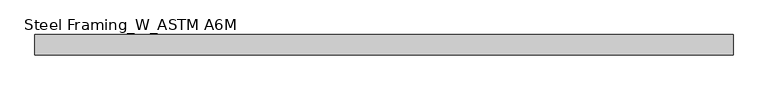
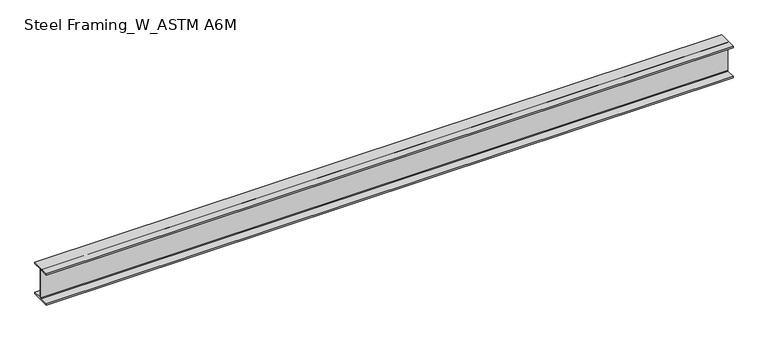
"""IFC4 building model written with IfcOpenShell, lengths in millimetres: beam geometry, Steel Framing_W_ASTM A6M : H_SB_AR_S02_W460x128_B1."""

from ifc_helpers import new_model, si_unit, point, frame, frame_2d, origin, place, context, project, spatial, polyline, circle_curve, trimmed, segment, composite_curve, outline, extrude, source, transform, mapped, element, save


def steel_framing_w_astm_a6m_6918b6cf(model_context):
    return source(origin(), model_context, "Body", "SweptSolid", [
        extrude(outline(composite_curve([segment(polyline([(141.0, -213.9), (141.0, -233.5), (-141.0, -233.5), (-141.0, -213.9), (-16.2, -213.9)]), True, "CONTINUOUS"), segment(trimmed(circle_curve(frame_2d((-16.2, -203.8)), 10.1), [point((-16.2, -213.9))], [point((-6.1, -203.8))], True, "CARTESIAN"), True, "CONTINUOUS"), segment(polyline([(-6.1, -203.8), (-6.1, 203.8)]), True, "CONTINUOUS"), segment(trimmed(circle_curve(frame_2d((-16.2, 203.8)), 10.1), [point((-6.1, 203.8))], [point((-16.2, 213.9))], True, "CARTESIAN"), True, "CONTINUOUS"), segment(polyline([(-16.2, 213.9), (-141.0, 213.9), (-141.0, 233.5), (141.0, 233.5), (141.0, 213.9), (16.2, 213.9)]), True, "CONTINUOUS"), segment(trimmed(circle_curve(frame_2d((16.2, 203.8)), 10.1), [point((16.2, 213.9))], [point((6.1, 203.8))], True, "CARTESIAN"), True, "CONTINUOUS"), segment(polyline([(6.1, 203.8), (6.1, -203.8)]), True, "CONTINUOUS"), segment(trimmed(circle_curve(frame_2d((16.2, -203.8)), 10.1), [point((6.1, -203.8))], [point((16.2, -213.9))], True, "CARTESIAN"), True, "CONTINUOUS"), segment(polyline([(16.2, -213.9), (141.0, -213.9)]), True, "CONTINUOUS")], self_intersect=False)), frame((-4846.3, 0.0, 0.0), z_axis=(1.0, 0.0, 0.0), x_axis=(0.0, 1.0, 0.0)), (0.0, 0.0, 1.0), 9692.6),
    ])


if __name__ == "__main__":
    model = new_model("IFC4")
    model_context = context("Model", 3, world=origin())
    ifc_project = project(units=[si_unit("LENGTHUNIT", "METRE", prefix="MILLI")], contexts=[model_context])
    site = spatial("IfcSite", under=ifc_project)
    building = spatial("IfcBuilding", under=site)
    placement = place(None, origin())
    steel_framing_w_astm_a6m_shape = steel_framing_w_astm_a6m_6918b6cf(model_context)
    element("IfcBeam", 1, ObjectType="Steel Framing_W_ASTM A6M : H_SB_AR_S02_W460x128_B1", at=placement, inside=building, context=model_context, shape_type="MappedRepresentation", body=[
        mapped(steel_framing_w_astm_a6m_shape, transform((0.0, 0.0, 0.0), x_axis=(1.0, 0.0, 0.0), y_axis=(0.0, 1.0, 0.0), z_axis=(0.0, 0.0, 1.0))),
    ])
    save(model, "model.ifc")

# Revit data of these elements
# Type "Steel Framing_W_ASTM A6M : H_SB_AR_S02_W460x128_B1"
#   Section Name Key = "W18x86"
#   Width = 28.2 cm
#   Web Thickness = 1.22 cm
#   Web Fillet = 1.01 cm
#   Warping Constant = 3650000.0 cm⁶
#   Torsional Moment of Inertia = 171.00 cm⁴
#   Section Area = 163.0 cm²
#   Plastic Modulus weak axis = 793.0 cm³
#   Plastic Modulus strong axis = 3050.0 cm³
#   Perimeter = 2.02 m²/m
#   Nominal Weight = 128.00 kgf/m
#   Moment of Inertia weak axis = 7280.00 cm⁴
#   Moment of Inertia strong axis = 63700.00 cm⁴
#   Height = 46.7 cm
#   Flange Thickness = 1.96 cm
#   Elastic Modulus weak axis = 518.0 cm³
#   Elastic Modulus strong axis = 2720.0 cm³
#   Centroid Vertical = 23.35 cm
#   Centroid Horizontal = 14.1 cm
#   Length [instance default] = 1500 mm
#   Structural Material [instance default] = Steel, 45-345
#   Bolt Spacing = 0
#   Assembly Code = ""
# Element 1 (IfcBeam, "Steel Framing_W_ASTM A6M : H_SB_AR_S02_W460x128_B1")
#   Materials on its faces: "Steel, 45-345"
# Materials
#   "Steel, 45-345": class "Metal", colour RGB 189 187 185, transparency 0, Description = "Steel 345 MPa", Cost = 0
